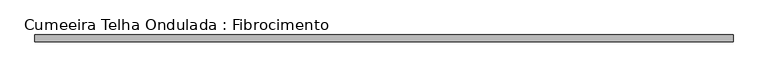
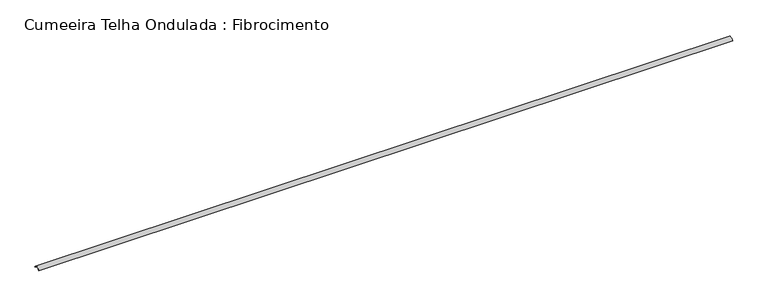
"""IFC4 building model written with IfcOpenShell, lengths in millimetres: beam geometry, Cumeeira Telha Ondulada : Fibrocimento."""

from ifc_helpers import new_model, si_unit, point, frame, frame_2d, origin, place, context, project, spatial, polyline, circle_curve, trimmed, segment, composite_curve, outline, extrude, source, transform, mapped, element, save


def cumeeira_telha_ondulada_fibrocimento_4a9e66c1(model_context):
    return source(origin(), model_context, "Body", "SweptSolid", [
        extrude(outline(composite_curve([segment(polyline([(58.3970135, 42.4437972), (53.9055884, 40.2467307)]), True, "CONTINUOUS"), segment(trimmed(circle_curve(frame_2d((-1.6029865, 13.0936483)), 61.7939461), [point((53.9055884, 40.2467307))], [point((-57.1115615, 40.2467307))], True, "CARTESIAN"), True, "CONTINUOUS"), segment(polyline([(-57.1115615, 40.2467307), (-61.6029865, 42.4437972)]), True, "CONTINUOUS"), segment(trimmed(circle_curve(frame_2d((-1.6029865, 13.0936483)), 66.7939461), [point((-61.6029865, 42.4437972))], [point((58.3970135, 42.4437972))], False, "CARTESIAN"), True, "CONTINUOUS")], self_intersect=False)), frame((-6200.0, 0.0, 0.0), z_axis=(1.0, 0.0, 0.0), x_axis=(0.0, 1.0, 0.0)), (0.0, 0.0, 1.0), 12400.0),
    ])


if __name__ == "__main__":
    model = new_model("IFC4")
    model_context = context("Model", 3, world=origin())
    ifc_project = project(units=[si_unit("LENGTHUNIT", "METRE", prefix="MILLI")], contexts=[model_context])
    site = spatial("IfcSite", under=ifc_project)
    building = spatial("IfcBuilding", under=site)
    placement = place(None, origin())
    cumeeira_telha_ondulada_fibrocimento_shape = cumeeira_telha_ondulada_fibrocimento_4a9e66c1(model_context)
    element("IfcBeam", 1, ObjectType="Cumeeira Telha Ondulada : Fibrocimento", at=placement, inside=building, context=model_context, shape_type="MappedRepresentation", body=[
        mapped(cumeeira_telha_ondulada_fibrocimento_shape, transform((0.0, 0.0, 0.0), x_axis=(1.0, 0.0, 0.0), y_axis=(0.0, 1.0, 0.0), z_axis=(0.0, 0.0, 1.0))),
    ])
    save(model, "model.ifc")

# Revit data of these elements
# Type "Cumeeira Telha Ondulada : Fibrocimento"
#   Cost = 5
#   Length [instance default] = 1.524 m
#   b = 0.07 m
#   h = 0.16 m
#   Structural Material = .TELHA DE FIBROCIMENTO
#   Assembly Code = ""
# Element 1 (IfcBeam, "Cumeeira Telha Ondulada : Fibrocimento")
#   Materials on its faces: ".TELHA DE FIBROCIMENTO"
# Materials
#   ".TELHA DE FIBROCIMENTO": class "CC_TELHADO", colour RGB 77 77 76, transparency 0, Description = "TELHA ONDULADA FIBROCIMENTO", Cost = 0
